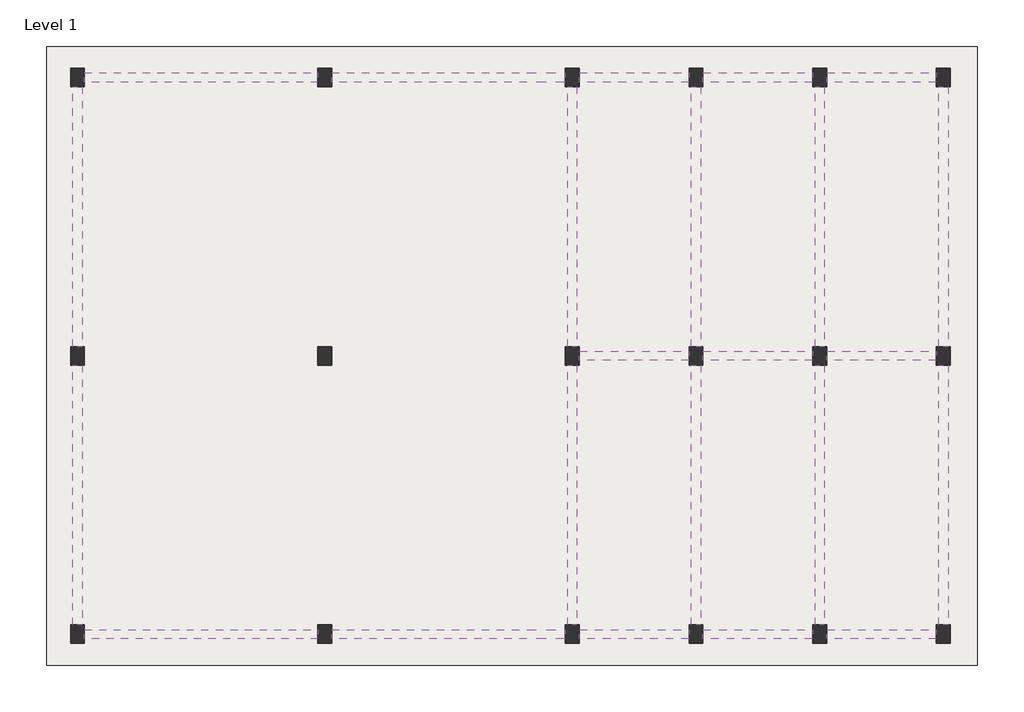
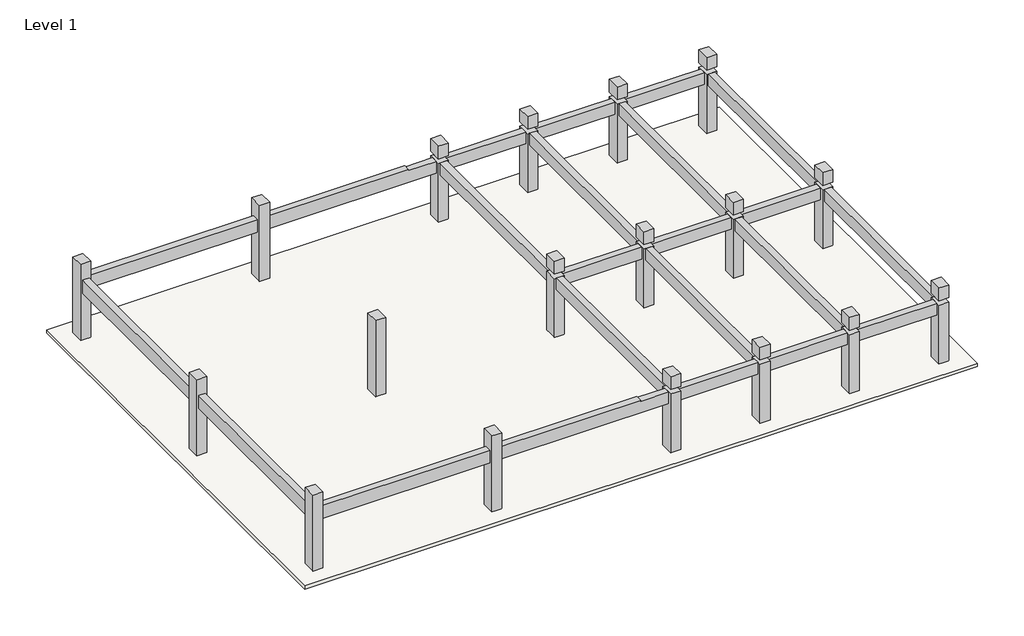
# One storey: 23 beams, 18 columns, 1 slab.
"""IFC4 building model written with IfcOpenShell, lengths in millimetres."""

from ifc_helpers import new_model, si_unit, frame, origin, origin_with_axes, place, context, project, spatial, polyline, outline, extrude, element, save

model = new_model("IFC4")

# Units and contexts
model_context = context("Model", 3, world=origin())
ifc_project = project(units=[si_unit("LENGTHUNIT", "METRE", prefix="MILLI")], contexts=[model_context])

# Site, building, storey
site = spatial("IfcSite", under=ifc_project)
building = spatial("IfcBuilding", under=site)
storey = spatial("IfcBuildingStorey", under=building, Name="Level 1", Elevation=0.0)

# Beams
placement = place(None, origin())
element("IfcBeam", 1, ObjectType="Concrete-Rectangular Beam : 300 x 600mm", at=placement, inside=storey, context=model_context, shape_type="SweptSolid", body=[
    extrude(outline(polyline([(-14991.2051668, 9433.1317199), (-14991.2051668, 9733.1317199), (-7441.2051668, 9733.1317199), (-7441.2051668, 9433.1317199), (-14991.2051668, 9433.1317199)])), frame((0.0, 0.0, 2240.0), z_axis=(0.0, 0.0, 1.0), x_axis=(1.0, 0.0, 0.0)), (0.0, 0.0, 1.0), 600.0),
])
element("IfcBeam", 2, ObjectType="Concrete-Rectangular Beam : 300 x 600mm", at=placement, inside=storey, context=model_context, shape_type="SweptSolid", body=[
    extrude(outline(polyline([(-14991.2051668, -8566.8682801), (-14991.2051668, -8266.8682801), (-7441.2051668, -8266.8682801), (-7441.2051668, -8566.8682801), (-14991.2051668, -8566.8682801)])), frame((0.0, 0.0, 2240.0), z_axis=(0.0, 0.0, 1.0), x_axis=(1.0, 0.0, 0.0)), (0.0, 0.0, 1.0), 600.0),
])
element("IfcBeam", 3, ObjectType="Concrete-Rectangular Beam : 300 x 600mm", at=placement, inside=storey, context=model_context, shape_type="SweptSolid", body=[
    extrude(outline(polyline([(2840.0, -6991.2051668), (2240.0, -6991.2051668), (2240.0, 558.7948332), (2785.0, 558.7948332), (2785.0, -687.3078946), (2840.0, -687.3078946), (2840.0, -6991.2051668)])), frame((0.0, -8566.8682801, 0.0), z_axis=(0.0, 1.0, 0.0), x_axis=(0.0, 0.0, 1.0)), (0.0, 0.0, 1.0), 300.0),
])
element("IfcBeam", 4, ObjectType="Concrete-Rectangular Beam : 300 x 600mm", at=placement, inside=storey, context=model_context, shape_type="SweptSolid", body=[
    extrude(outline(polyline([(1008.7948332, -8566.8682801), (1008.7948332, -8266.8682801), (4558.7948332, -8266.8682801), (4558.7948332, -8566.8682801), (1008.7948332, -8566.8682801)])), frame((0.0, 0.0, 2240.0), z_axis=(0.0, 0.0, 1.0), x_axis=(1.0, 0.0, 0.0)), (0.0, 0.0, 1.0), 545.0),
])
element("IfcBeam", 5, ObjectType="Concrete-Rectangular Beam : 300 x 600mm", at=placement, inside=storey, context=model_context, shape_type="SweptSolid", body=[
    extrude(outline(polyline([(8558.7948332, -8266.8682801), (8558.7948332, -8566.8682801), (5008.7948332, -8566.8682801), (5008.7948332, -8266.8682801), (8558.7948332, -8266.8682801)])), frame((0.0, 0.0, 2240.0), z_axis=(0.0, 0.0, 1.0), x_axis=(1.0, 0.0, 0.0)), (0.0, 0.0, 1.0), 545.0),
])
element("IfcBeam", 6, ObjectType="Concrete-Rectangular Beam : 300 x 600mm", at=placement, inside=storey, context=model_context, shape_type="SweptSolid", body=[
    extrude(outline(polyline([(9008.7948332, -8566.8682801), (9008.7948332, -8266.8682801), (12558.7948332, -8266.8682801), (12558.7948332, -8566.8682801), (9008.7948332, -8566.8682801)])), frame((0.0, 0.0, 2240.0), z_axis=(0.0, 0.0, 1.0), x_axis=(1.0, 0.0, 0.0)), (0.0, 0.0, 1.0), 545.0),
])
element("IfcBeam", 7, ObjectType="Concrete-Rectangular Beam : 300 x 600mm", at=placement, inside=storey, context=model_context, shape_type="SweptSolid", body=[
    extrude(outline(polyline([(12633.7948332, 283.1317199), (12933.7948332, 283.1317199), (12933.7948332, -8116.8682801), (12633.7948332, -8116.8682801), (12633.7948332, 283.1317199)])), frame((0.0, 0.0, 2240.0), z_axis=(0.0, 0.0, 1.0), x_axis=(1.0, 0.0, 0.0)), (0.0, 0.0, 1.0), 545.0),
])
element("IfcBeam", 8, ObjectType="Concrete-Rectangular Beam : 300 x 600mm", at=placement, inside=storey, context=model_context, shape_type="SweptSolid", body=[
    extrude(outline(polyline([(12633.7948332, 9283.1317199), (12933.7948332, 9283.1317199), (12933.7948332, 883.1317199), (12633.7948332, 883.1317199), (12633.7948332, 9283.1317199)])), frame((0.0, 0.0, 2240.0), z_axis=(0.0, 0.0, 1.0), x_axis=(1.0, 0.0, 0.0)), (0.0, 0.0, 1.0), 545.0),
])
element("IfcBeam", 9, ObjectType="Concrete-Rectangular Beam : 300 x 600mm", at=placement, inside=storey, context=model_context, shape_type="SweptSolid", body=[
    extrude(outline(polyline([(8933.7948332, 883.1317199), (8633.7948332, 883.1317199), (8633.7948332, 9283.1317199), (8933.7948332, 9283.1317199), (8933.7948332, 883.1317199)])), frame((0.0, 0.0, 2240.0), z_axis=(0.0, 0.0, 1.0), x_axis=(1.0, 0.0, 0.0)), (0.0, 0.0, 1.0), 545.0),
])
element("IfcBeam", 10, ObjectType="Concrete-Rectangular Beam : 300 x 600mm", at=placement, inside=storey, context=model_context, shape_type="SweptSolid", body=[
    extrude(outline(polyline([(4933.7948332, 883.1317199), (4633.7948332, 883.1317199), (4633.7948332, 9283.1317199), (4933.7948332, 9283.1317199), (4933.7948332, 883.1317199)])), frame((0.0, 0.0, 2240.0), z_axis=(0.0, 0.0, 1.0), x_axis=(1.0, 0.0, 0.0)), (0.0, 0.0, 1.0), 545.0),
])
element("IfcBeam", 11, ObjectType="Concrete-Rectangular Beam : 300 x 600mm", at=placement, inside=storey, context=model_context, shape_type="SweptSolid", body=[
    extrude(outline(polyline([(633.7948332, 9283.1317199), (933.7948332, 9283.1317199), (933.7948332, 883.1317199), (633.7948332, 883.1317199), (633.7948332, 9283.1317199)])), frame((0.0, 0.0, 2240.0), z_axis=(0.0, 0.0, 1.0), x_axis=(1.0, 0.0, 0.0)), (0.0, 0.0, 1.0), 545.0),
])
element("IfcBeam", 12, ObjectType="Concrete-Rectangular Beam : 300 x 600mm", at=placement, inside=storey, context=model_context, shape_type="SweptSolid", body=[
    extrude(outline(polyline([(633.7948332, 283.1317199), (933.7948332, 283.1317199), (933.7948332, -8116.8682801), (633.7948332, -8116.8682801), (633.7948332, 283.1317199)])), frame((0.0, 0.0, 2240.0), z_axis=(0.0, 0.0, 1.0), x_axis=(1.0, 0.0, 0.0)), (0.0, 0.0, 1.0), 545.0),
])
element("IfcBeam", 13, ObjectType="Concrete-Rectangular Beam : 300 x 600mm", at=placement, inside=storey, context=model_context, shape_type="SweptSolid", body=[
    extrude(outline(polyline([(4933.7948332, -8116.8682801), (4633.7948332, -8116.8682801), (4633.7948332, 283.1317199), (4933.7948332, 283.1317199), (4933.7948332, -8116.8682801)])), frame((0.0, 0.0, 2240.0), z_axis=(0.0, 0.0, 1.0), x_axis=(1.0, 0.0, 0.0)), (0.0, 0.0, 1.0), 545.0),
])
element("IfcBeam", 14, ObjectType="Concrete-Rectangular Beam : 300 x 600mm", at=placement, inside=storey, context=model_context, shape_type="SweptSolid", body=[
    extrude(outline(polyline([(8933.7948332, -8116.8682801), (8633.7948332, -8116.8682801), (8633.7948332, 283.1317199), (8933.7948332, 283.1317199), (8933.7948332, -8116.8682801)])), frame((0.0, 0.0, 2240.0), z_axis=(0.0, 0.0, 1.0), x_axis=(1.0, 0.0, 0.0)), (0.0, 0.0, 1.0), 545.0),
])
element("IfcBeam", 15, ObjectType="Concrete-Rectangular Beam : 300 x 600mm", at=placement, inside=storey, context=model_context, shape_type="SweptSolid", body=[
    extrude(outline(polyline([(2840.0, -6991.2051668), (2240.0, -6991.2051668), (2240.0, 558.7948332), (2785.0, 558.7948332), (2785.0, -687.3078946), (2840.0, -687.3078946), (2840.0, -6991.2051668)])), frame((0.0, 9433.1317199, 0.0), z_axis=(0.0, 1.0, 0.0), x_axis=(0.0, 0.0, 1.0)), (0.0, 0.0, 1.0), 300.0),
])
element("IfcBeam", 16, ObjectType="Concrete-Rectangular Beam : 300 x 600mm", at=placement, inside=storey, context=model_context, shape_type="SweptSolid", body=[
    extrude(outline(polyline([(-15366.2051668, 9283.1317199), (-15066.2051668, 9283.1317199), (-15066.2051668, 883.1317199), (-15366.2051668, 883.1317199), (-15366.2051668, 9283.1317199)])), frame((0.0, 0.0, 2240.0), z_axis=(0.0, 0.0, 1.0), x_axis=(1.0, 0.0, 0.0)), (0.0, 0.0, 1.0), 600.0),
])
element("IfcBeam", 17, ObjectType="Concrete-Rectangular Beam : 300 x 600mm", at=placement, inside=storey, context=model_context, shape_type="SweptSolid", body=[
    extrude(outline(polyline([(-15366.2051668, 283.1317199), (-15066.2051668, 283.1317199), (-15066.2051668, -8116.8682801), (-15366.2051668, -8116.8682801), (-15366.2051668, 283.1317199)])), frame((0.0, 0.0, 2240.0), z_axis=(0.0, 0.0, 1.0), x_axis=(1.0, 0.0, 0.0)), (0.0, 0.0, 1.0), 600.0),
])
element("IfcBeam", 18, ObjectType="Concrete-Rectangular Beam : 300 x 600mm", at=placement, inside=storey, context=model_context, shape_type="SweptSolid", body=[
    extrude(outline(polyline([(1008.7948332, 9433.1317199), (1008.7948332, 9733.1317199), (4558.7948332, 9733.1317199), (4558.7948332, 9433.1317199), (1008.7948332, 9433.1317199)])), frame((0.0, 0.0, 2240.0), z_axis=(0.0, 0.0, 1.0), x_axis=(1.0, 0.0, 0.0)), (0.0, 0.0, 1.0), 545.0),
])
element("IfcBeam", 19, ObjectType="Concrete-Rectangular Beam : 300 x 600mm", at=placement, inside=storey, context=model_context, shape_type="SweptSolid", body=[
    extrude(outline(polyline([(8558.7948332, 9733.1317199), (8558.7948332, 9433.1317199), (5008.7948332, 9433.1317199), (5008.7948332, 9733.1317199), (8558.7948332, 9733.1317199)])), frame((0.0, 0.0, 2240.0), z_axis=(0.0, 0.0, 1.0), x_axis=(1.0, 0.0, 0.0)), (0.0, 0.0, 1.0), 545.0),
])
element("IfcBeam", 20, ObjectType="Concrete-Rectangular Beam : 300 x 600mm", at=placement, inside=storey, context=model_context, shape_type="SweptSolid", body=[
    extrude(outline(polyline([(9008.7948332, 9433.1317199), (9008.7948332, 9733.1317199), (12558.7948332, 9733.1317199), (12558.7948332, 9433.1317199), (9008.7948332, 9433.1317199)])), frame((0.0, 0.0, 2240.0), z_axis=(0.0, 0.0, 1.0), x_axis=(1.0, 0.0, 0.0)), (0.0, 0.0, 1.0), 545.0),
])
element("IfcBeam", 21, ObjectType="Concrete-Rectangular Beam : 300 x 600mm", at=placement, inside=storey, context=model_context, shape_type="SweptSolid", body=[
    extrude(outline(polyline([(1008.7948332, 433.1317199), (1008.7948332, 733.1317199), (4558.7948332, 733.1317199), (4558.7948332, 433.1317199), (1008.7948332, 433.1317199)])), frame((0.0, 0.0, 2240.0), z_axis=(0.0, 0.0, 1.0), x_axis=(1.0, 0.0, 0.0)), (0.0, 0.0, 1.0), 545.0),
])
element("IfcBeam", 22, ObjectType="Concrete-Rectangular Beam : 300 x 600mm", at=placement, inside=storey, context=model_context, shape_type="SweptSolid", body=[
    extrude(outline(polyline([(8558.7948332, 733.1317199), (8558.7948332, 433.1317199), (5008.7948332, 433.1317199), (5008.7948332, 733.1317199), (8558.7948332, 733.1317199)])), frame((0.0, 0.0, 2240.0), z_axis=(0.0, 0.0, 1.0), x_axis=(1.0, 0.0, 0.0)), (0.0, 0.0, 1.0), 545.0),
])
element("IfcBeam", 23, ObjectType="Concrete-Rectangular Beam : 300 x 600mm", at=placement, inside=storey, context=model_context, shape_type="SweptSolid", body=[
    extrude(outline(polyline([(9008.7948332, 433.1317199), (9008.7948332, 733.1317199), (12558.7948332, 733.1317199), (12558.7948332, 433.1317199), (9008.7948332, 433.1317199)])), frame((0.0, 0.0, 2240.0), z_axis=(0.0, 0.0, 1.0), x_axis=(1.0, 0.0, 0.0)), (0.0, 0.0, 1.0), 545.0),
])

# Columns
element("IfcColumn", 24, ObjectType="Concrete-Rectangular-Column : 450 x 600mm", at=placement, inside=storey, context=model_context, shape_type="SweptSolid", body=[
    extrude(outline(polyline([(-14991.2051668, 9883.1317199), (-14991.2051668, 9283.1317199), (-15441.2051668, 9283.1317199), (-15441.2051668, 9883.1317199), (-14991.2051668, 9883.1317199)])), origin_with_axes(), (0.0, 0.0, 1.0), 3600.0),
])
element("IfcColumn", 25, ObjectType="Concrete-Rectangular-Column : 450 x 600mm", at=placement, inside=storey, context=model_context, shape_type="SweptSolid", body=[
    extrude(outline(polyline([(-14991.2051668, 883.1317199), (-14991.2051668, 283.1317199), (-15441.2051668, 283.1317199), (-15441.2051668, 883.1317199), (-14991.2051668, 883.1317199)])), origin_with_axes(), (0.0, 0.0, 1.0), 3600.0),
])
element("IfcColumn", 26, ObjectType="Concrete-Rectangular-Column : 450 x 600mm", at=placement, inside=storey, context=model_context, shape_type="SweptSolid", body=[
    extrude(outline(polyline([(-14991.2051668, -8116.8682801), (-14991.2051668, -8716.8682801), (-15441.2051668, -8716.8682801), (-15441.2051668, -8116.8682801), (-14991.2051668, -8116.8682801)])), origin_with_axes(), (0.0, 0.0, 1.0), 3600.0),
])
element("IfcColumn", 27, ObjectType="Concrete-Rectangular-Column : 450 x 600mm", at=placement, inside=storey, context=model_context, shape_type="SweptSolid", body=[
    extrude(outline(polyline([(-6991.2051668, -8116.8682801), (-6991.2051668, -8716.8682801), (-7441.2051668, -8716.8682801), (-7441.2051668, -8116.8682801), (-6991.2051668, -8116.8682801)])), origin_with_axes(), (0.0, 0.0, 1.0), 3600.0),
])
element("IfcColumn", 28, ObjectType="Concrete-Rectangular-Column : 450 x 600mm", at=placement, inside=storey, context=model_context, shape_type="SweptSolid", body=[
    extrude(outline(polyline([(-6991.2051668, 883.1317199), (-6991.2051668, 283.1317199), (-7441.2051668, 283.1317199), (-7441.2051668, 883.1317199), (-6991.2051668, 883.1317199)])), origin_with_axes(), (0.0, 0.0, 1.0), 3600.0),
])
element("IfcColumn", 29, ObjectType="Concrete-Rectangular-Column : 450 x 600mm", at=placement, inside=storey, context=model_context, shape_type="SweptSolid", body=[
    extrude(outline(polyline([(-6991.2051668, 9883.1317199), (-6991.2051668, 9283.1317199), (-7441.2051668, 9283.1317199), (-7441.2051668, 9883.1317199), (-6991.2051668, 9883.1317199)])), origin_with_axes(), (0.0, 0.0, 1.0), 3600.0),
])
element("IfcColumn", 30, ObjectType="Concrete-Rectangular-Column : 450 x 600mm", at=placement, inside=storey, context=model_context, shape_type="SweptSolid", body=[
    extrude(outline(polyline([(558.7948332, 9883.1317199), (1008.7948332, 9883.1317199), (1008.7948332, 9283.1317199), (558.7948332, 9283.1317199), (558.7948332, 9883.1317199)])), frame((0.0, 0.0, 3000.0), z_axis=(0.0, 0.0, 1.0), x_axis=(1.0, 0.0, 0.0)), (0.0, 0.0, 1.0), 600.0),
    extrude(outline(polyline([(1008.7948332, 9883.1317199), (1008.7948332, 9283.1317199), (558.7948332, 9283.1317199), (558.7948332, 9883.1317199), (1008.7948332, 9883.1317199)])), origin_with_axes(), (0.0, 0.0, 1.0), 2785.0),
])
element("IfcColumn", 31, ObjectType="Concrete-Rectangular-Column : 450 x 600mm", at=placement, inside=storey, context=model_context, shape_type="SweptSolid", body=[
    extrude(outline(polyline([(558.7948332, 883.1317199), (1008.7948332, 883.1317199), (1008.7948332, 283.1317199), (558.7948332, 283.1317199), (558.7948332, 883.1317199)])), frame((0.0, 0.0, 3000.0), z_axis=(0.0, 0.0, 1.0), x_axis=(1.0, 0.0, 0.0)), (0.0, 0.0, 1.0), 600.0),
    extrude(outline(polyline([(1008.7948332, 883.1317199), (1008.7948332, 283.1317199), (558.7948332, 283.1317199), (558.7948332, 883.1317199), (1008.7948332, 883.1317199)])), origin_with_axes(), (0.0, 0.0, 1.0), 2785.0),
])
element("IfcColumn", 32, ObjectType="Concrete-Rectangular-Column : 450 x 600mm", at=placement, inside=storey, context=model_context, shape_type="SweptSolid", body=[
    extrude(outline(polyline([(558.7948332, -8116.8682801), (1008.7948332, -8116.8682801), (1008.7948332, -8716.8682801), (558.7948332, -8716.8682801), (558.7948332, -8116.8682801)])), frame((0.0, 0.0, 3000.0), z_axis=(0.0, 0.0, 1.0), x_axis=(1.0, 0.0, 0.0)), (0.0, 0.0, 1.0), 600.0),
    extrude(outline(polyline([(1008.7948332, -8116.8682801), (1008.7948332, -8716.8682801), (558.7948332, -8716.8682801), (558.7948332, -8116.8682801), (1008.7948332, -8116.8682801)])), origin_with_axes(), (0.0, 0.0, 1.0), 2785.0),
])
element("IfcColumn", 33, ObjectType="Concrete-Rectangular-Column : 450 x 600mm", at=placement, inside=storey, context=model_context, shape_type="SweptSolid", body=[
    extrude(outline(polyline([(8558.7948332, -8116.8682801), (9008.7948332, -8116.8682801), (9008.7948332, -8716.8682801), (8558.7948332, -8716.8682801), (8558.7948332, -8116.8682801)])), frame((0.0, 0.0, 3000.0), z_axis=(0.0, 0.0, 1.0), x_axis=(1.0, 0.0, 0.0)), (0.0, 0.0, 1.0), 600.0),
    extrude(outline(polyline([(9008.7948332, -8116.8682801), (9008.7948332, -8716.8682801), (8558.7948332, -8716.8682801), (8558.7948332, -8116.8682801), (9008.7948332, -8116.8682801)])), origin_with_axes(), (0.0, 0.0, 1.0), 2785.0),
])
element("IfcColumn", 34, ObjectType="Concrete-Rectangular-Column : 450 x 600mm", at=placement, inside=storey, context=model_context, shape_type="SweptSolid", body=[
    extrude(outline(polyline([(8558.7948332, 883.1317199), (9008.7948332, 883.1317199), (9008.7948332, 283.1317199), (8558.7948332, 283.1317199), (8558.7948332, 883.1317199)])), frame((0.0, 0.0, 3000.0), z_axis=(0.0, 0.0, 1.0), x_axis=(1.0, 0.0, 0.0)), (0.0, 0.0, 1.0), 600.0),
    extrude(outline(polyline([(9008.7948332, 883.1317199), (9008.7948332, 283.1317199), (8558.7948332, 283.1317199), (8558.7948332, 883.1317199), (9008.7948332, 883.1317199)])), origin_with_axes(), (0.0, 0.0, 1.0), 2785.0),
])
element("IfcColumn", 35, ObjectType="Concrete-Rectangular-Column : 450 x 600mm", at=placement, inside=storey, context=model_context, shape_type="SweptSolid", body=[
    extrude(outline(polyline([(8558.7948332, 9883.1317199), (9008.7948332, 9883.1317199), (9008.7948332, 9283.1317199), (8558.7948332, 9283.1317199), (8558.7948332, 9883.1317199)])), frame((0.0, 0.0, 3000.0), z_axis=(0.0, 0.0, 1.0), x_axis=(1.0, 0.0, 0.0)), (0.0, 0.0, 1.0), 600.0),
    extrude(outline(polyline([(9008.7948332, 9883.1317199), (9008.7948332, 9283.1317199), (8558.7948332, 9283.1317199), (8558.7948332, 9883.1317199), (9008.7948332, 9883.1317199)])), origin_with_axes(), (0.0, 0.0, 1.0), 2785.0),
])
element("IfcColumn", 36, ObjectType="Concrete-Rectangular-Column : 450 x 600mm", at=placement, inside=storey, context=model_context, shape_type="SweptSolid", body=[
    extrude(outline(polyline([(12558.7948332, 9883.1317199), (13008.7948332, 9883.1317199), (13008.7948332, 9283.1317199), (12558.7948332, 9283.1317199), (12558.7948332, 9883.1317199)])), frame((0.0, 0.0, 3000.0), z_axis=(0.0, 0.0, 1.0), x_axis=(1.0, 0.0, 0.0)), (0.0, 0.0, 1.0), 600.0),
    extrude(outline(polyline([(13008.7948332, 9883.1317199), (13008.7948332, 9283.1317199), (12558.7948332, 9283.1317199), (12558.7948332, 9883.1317199), (13008.7948332, 9883.1317199)])), origin_with_axes(), (0.0, 0.0, 1.0), 2785.0),
])
element("IfcColumn", 37, ObjectType="Concrete-Rectangular-Column : 450 x 600mm", at=placement, inside=storey, context=model_context, shape_type="SweptSolid", body=[
    extrude(outline(polyline([(12558.7948332, 883.1317199), (13008.7948332, 883.1317199), (13008.7948332, 283.1317199), (12558.7948332, 283.1317199), (12558.7948332, 883.1317199)])), frame((0.0, 0.0, 3000.0), z_axis=(0.0, 0.0, 1.0), x_axis=(1.0, 0.0, 0.0)), (0.0, 0.0, 1.0), 600.0),
    extrude(outline(polyline([(13008.7948332, 883.1317199), (13008.7948332, 283.1317199), (12558.7948332, 283.1317199), (12558.7948332, 883.1317199), (13008.7948332, 883.1317199)])), origin_with_axes(), (0.0, 0.0, 1.0), 2785.0),
])
element("IfcColumn", 38, ObjectType="Concrete-Rectangular-Column : 450 x 600mm", at=placement, inside=storey, context=model_context, shape_type="SweptSolid", body=[
    extrude(outline(polyline([(12558.7948332, -8116.8682801), (13008.7948332, -8116.8682801), (13008.7948332, -8716.8682801), (12558.7948332, -8716.8682801), (12558.7948332, -8116.8682801)])), frame((0.0, 0.0, 3000.0), z_axis=(0.0, 0.0, 1.0), x_axis=(1.0, 0.0, 0.0)), (0.0, 0.0, 1.0), 600.0),
    extrude(outline(polyline([(13008.7948332, -8116.8682801), (13008.7948332, -8716.8682801), (12558.7948332, -8716.8682801), (12558.7948332, -8116.8682801), (13008.7948332, -8116.8682801)])), origin_with_axes(), (0.0, 0.0, 1.0), 2785.0),
])
element("IfcColumn", 39, ObjectType="Concrete-Rectangular-Column : 450 x 600mm", at=placement, inside=storey, context=model_context, shape_type="SweptSolid", body=[
    extrude(outline(polyline([(4558.7948332, -8116.8682801), (5008.7948332, -8116.8682801), (5008.7948332, -8716.8682801), (4558.7948332, -8716.8682801), (4558.7948332, -8116.8682801)])), frame((0.0, 0.0, 3000.0), z_axis=(0.0, 0.0, 1.0), x_axis=(1.0, 0.0, 0.0)), (0.0, 0.0, 1.0), 600.0),
    extrude(outline(polyline([(5008.7948332, -8116.8682801), (5008.7948332, -8716.8682801), (4558.7948332, -8716.8682801), (4558.7948332, -8116.8682801), (5008.7948332, -8116.8682801)])), origin_with_axes(), (0.0, 0.0, 1.0), 2785.0),
])
element("IfcColumn", 40, ObjectType="Concrete-Rectangular-Column : 450 x 600mm", at=placement, inside=storey, context=model_context, shape_type="SweptSolid", body=[
    extrude(outline(polyline([(4558.7948332, 883.1317199), (5008.7948332, 883.1317199), (5008.7948332, 283.1317199), (4558.7948332, 283.1317199), (4558.7948332, 883.1317199)])), frame((0.0, 0.0, 3000.0), z_axis=(0.0, 0.0, 1.0), x_axis=(1.0, 0.0, 0.0)), (0.0, 0.0, 1.0), 600.0),
    extrude(outline(polyline([(5008.7948332, 883.1317199), (5008.7948332, 283.1317199), (4558.7948332, 283.1317199), (4558.7948332, 883.1317199), (5008.7948332, 883.1317199)])), origin_with_axes(), (0.0, 0.0, 1.0), 2785.0),
])
element("IfcColumn", 41, ObjectType="Concrete-Rectangular-Column : 450 x 600mm", at=placement, inside=storey, context=model_context, shape_type="SweptSolid", body=[
    extrude(outline(polyline([(4558.7948332, 9883.1317199), (5008.7948332, 9883.1317199), (5008.7948332, 9283.1317199), (4558.7948332, 9283.1317199), (4558.7948332, 9883.1317199)])), frame((0.0, 0.0, 3000.0), z_axis=(0.0, 0.0, 1.0), x_axis=(1.0, 0.0, 0.0)), (0.0, 0.0, 1.0), 600.0),
    extrude(outline(polyline([(5008.7948332, 9883.1317199), (5008.7948332, 9283.1317199), (4558.7948332, 9283.1317199), (4558.7948332, 9883.1317199), (5008.7948332, 9883.1317199)])), origin_with_axes(), (0.0, 0.0, 1.0), 2785.0),
])

# Slab
element("IfcSlab", 42, ObjectType="150mm Foundation Slab", at=placement, inside=storey, context=model_context, shape_type="SweptSolid", body=[
    extrude(outline(polyline([(13883.7948332, 10583.1317199), (13883.7948332, -9416.8682801), (-16216.2051668, -9416.8682801), (-16216.2051668, 10583.1317199), (13883.7948332, 10583.1317199)])), frame((0.0, 0.0, -150.0), z_axis=(0.0, 0.0, 1.0), x_axis=(1.0, 0.0, 0.0)), (0.0, 0.0, 1.0), 150.0),
])

save(model, "model.ifc")

# Revit data of these elements
# Project information
#   Project Issue Date = "Issue Date"
#   Project Status = "Project Status"
#   Client Name = "Owner"
#   Project Address = "Enter address here"
#   Project Name = "Project Name"
#   Project Number = "Project Number"
# Grids (mm)
#   "1": line (-15216.205, 15561.914) -> (-15216.205, -13947.862)
#   "2": line (-11216.205, 15561.914) -> (-11216.205, -13947.862)
#   "3": line (-7216.205, 15561.914) -> (-7216.205, -13947.862)
#   "4": line (-3216.205, 15561.914) -> (-3216.205, -13947.862)
#   "5": line (783.795, 15561.914) -> (783.795, -13947.862)
#   "6": line (4783.795, 15561.914) -> (4783.795, -13947.862)
#   "7": line (8783.795, 15561.914) -> (8783.795, -13947.862)
#   "8": line (12783.795, 15561.914) -> (12783.795, -13947.862)
#   "A": line (-19643.464, 9583.132) -> (12783.795, 9583.132)
#   "B": line (-19643.464, 6583.132) -> (12783.795, 6583.132)
#   "C": line (-19643.464, 3583.132) -> (12783.795, 3583.132)
#   "D": line (-19643.464, 583.132) -> (12783.795, 583.132)
#   "E": line (-19643.464, -2416.868) -> (12783.795, -2416.868)
#   "F": line (-19643.464, -5416.868) -> (12783.795, -5416.868)
#   "G": line (-19643.464, -8416.868) -> (12783.795, -8416.868)
# Type "Concrete-Rectangular Beam : 300 x 600mm"
#   Length [instance default] = 1524 mm
#   b = 300 mm
#   h = 600 mm
#   Structural Material [instance default] = Concrete, Cast-in-Place gray
#   Assembly Code = ""
# Type "Concrete-Rectangular-Column : 450 x 600mm"
#   b = 450 mm
#   h = 600 mm
#   Structural Material [instance default] = Concrete, Cast-in-Place gray
# Type "150mm Foundation Slab"
#   Layers, outside or top first: 150 mm "Concrete, Cast-in-Place gray" (function 1)
# Elements 1, 2, 3, 4, 5, 6, 7, 8, 9, 10, 11, 12, 13, 14, 15, 16, 17, 18, 19, 20, 21, 22, 23 (IfcBeam, "Concrete-Rectangular Beam : 300 x 600mm")
#   Structural Material = Concrete, Cast-in-Place gray
#   Phase Created = New Construction
#   Materials on its faces: "Concrete, Cast-in-Place gray"
# Elements 24, 25, 26, 27, 28, 29, 30, 31, 32, 33, 34, 35, 36, 37, 38, 39, 40, 41 (IfcColumn, "Concrete-Rectangular-Column : 450 x 600mm")
#   Structural Material = Concrete, Cast-in-Place gray
#   Phase Created = New Construction
#   Materials on its faces: "Concrete, Cast-in-Place gray"
# Element 42 (IfcSlab, "150mm Foundation Slab")
#   Height Offset From Level = 0 mm
#   built-in parameter 1001954 = 1
#   Phase Created = New Construction
#   Materials on its faces: "Concrete, Cast-in-Place gray"
# Materials
#   "Concrete, Cast-in-Place gray": class "Concrete", colour RGB 192 192 192, transparency 0, Description = "Cast-in-place concrete", Cost = 0
